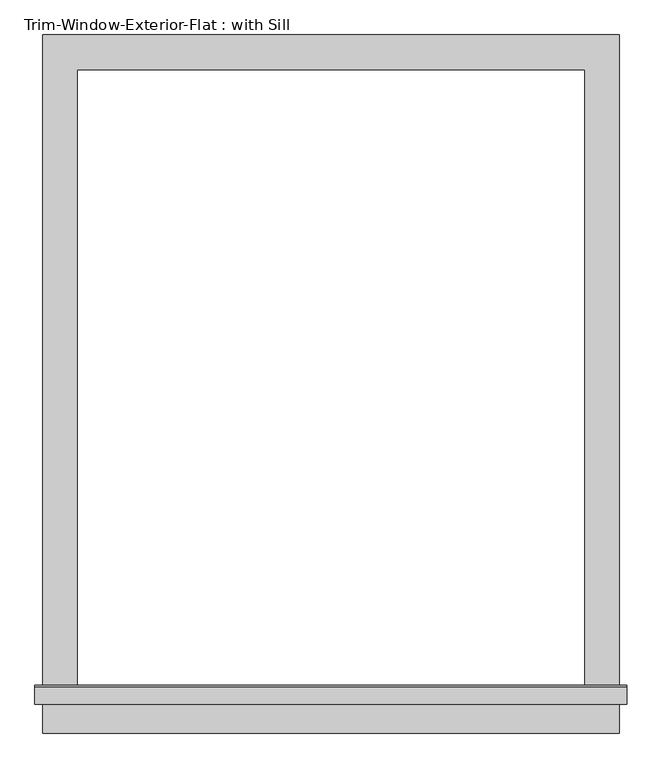
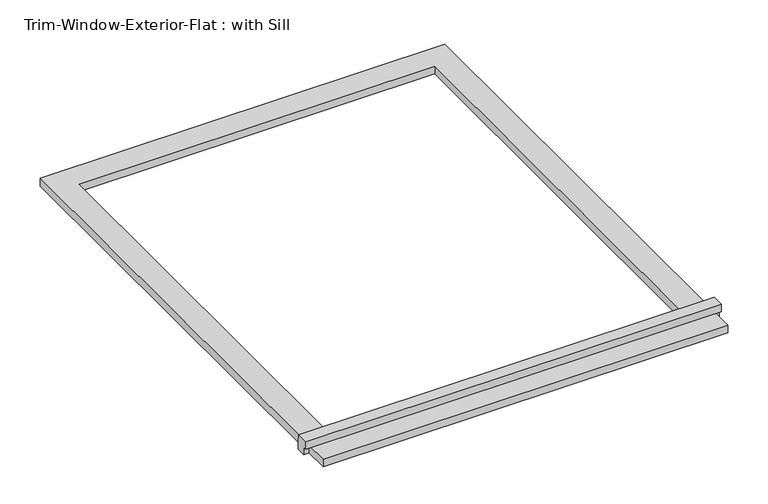
"""IFC4 building model written with IfcOpenShell, lengths in millimetres: proxy geometry, Trim-Window-Exterior-Flat : with Sill."""

from ifc_helpers import new_model, si_unit, frame, origin, origin_with_axes, place, context, project, spatial, polyline, outline, extrude, source, transform, mapped, element, save


def trim_window_exterior_flat_with_sill_d0c475a0(model_context):
    return source(origin(), model_context, "Body", "SweptSolid", [
        extrude(outline(polyline([(476.25, -1038.1823709), (476.25, -1095.3323709), (-476.25, -1095.3323709), (-476.25, -1038.1823709), (476.25, -1038.1823709)])), origin_with_axes(), (0.0, 0.0, 1.0), 19.05),
        extrude(outline(polyline([(-1047.75, 38.1), (-1018.4580645, 38.1), (-1016.0, 19.05), (-1016.0, 0.0), (-1038.1823709, 0.0), (-1038.1823709, 19.05), (-1047.75, 19.05), (-1047.75, 38.1)])), frame((-488.95, 0.0, 0.0), z_axis=(1.0, 0.0, 0.0), x_axis=(0.0, 1.0, 0.0)), (0.0, 0.0, 1.0), 977.9),
        extrude(outline(polyline([(-476.25, 57.15), (476.25, 57.15), (476.25, -1016.0), (419.1, -1016.0), (419.1, 0.0), (-419.1, 0.0), (-419.1, -1016.0), (-476.25, -1016.0), (-476.25, 57.15)])), origin_with_axes(), (0.0, 0.0, 1.0), 19.05),
    ])


if __name__ == "__main__":
    model = new_model("IFC4")
    model_context = context("Model", 3, world=origin())
    ifc_project = project(units=[si_unit("LENGTHUNIT", "METRE", prefix="MILLI")], contexts=[model_context])
    site = spatial("IfcSite", under=ifc_project)
    building = spatial("IfcBuilding", under=site)
    placement = place(None, origin())
    trim_window_exterior_flat_with_sill_shape = trim_window_exterior_flat_with_sill_d0c475a0(model_context)
    element("IfcBuildingElementProxy", 1, Name="Trim-Window-Exterior-Flat : with Sill", ObjectType="Trim-Window-Exterior-Flat : with Sill", at=placement, inside=building, context=model_context, shape_type="MappedRepresentation", body=[
        mapped(trim_window_exterior_flat_with_sill_shape, transform((0.0, 0.0, 0.0), x_axis=(1.0, 0.0, 0.0), y_axis=(0.0, 1.0, 0.0), z_axis=(0.0, 0.0, 1.0))),
    ])
    save(model, "model.ifc")

# Revit data of these elements
# Type "Trim-Window-Exterior-Flat : with Sill"
#   Trim Width = 0' - 2 1/4"
#   Trim Thickness_Picture Frame = 0' - 1 1/4"
#   Trim Thickness_with Sill = 0' - 0 3/4"
#   Sill Thickness = 0' - 1 1/4"
#   Opening Width [instance default] = 2' - 0"
#   Opening Height [instance default] = 3' - 0"
#   Default Elevation = 4' - 0"
#   Sill = yes
#   Picture Frame = no
#   Trim Material [instance default] = none
# Element 1 (IfcBuildingElementProxy, "Trim-Window-Exterior-Flat : with Sill")
#   Opening Width = 2' - 9"
#   Opening Height = 3' - 4"
#   Trim Material = 1X WOOD COMPOSITE TRIM
#   Materials on its faces: "1X WOOD COMPOSITE TRIM"
# Materials
#   "1X WOOD COMPOSITE TRIM": class "Generic", colour RGB 88 61 61, transparency 0, Cost = 0
